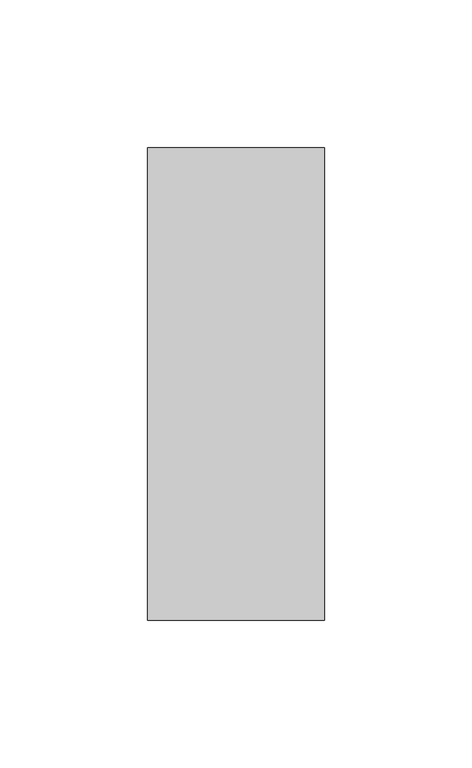
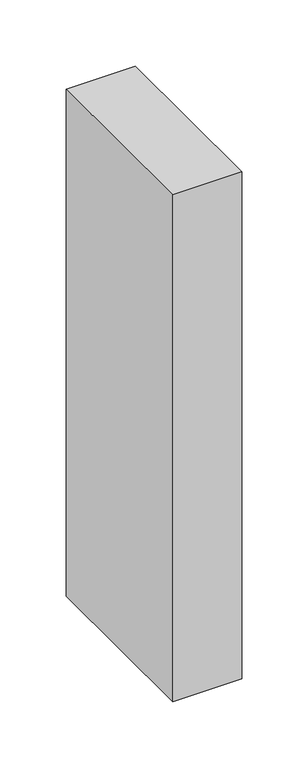
"""IFC4 building model written with IfcOpenShell, lengths in millimetres: column geometry, Madeira de lei-Coluna : Pontalete 6X16cm."""

import ifcopenshell
import ifcopenshell.guid

model = None  # the IFC model being written
_history = None  # IfcOwnerHistory: only IFC2X3 demands one
_inside = {}  # id of a spatial element -> (the spatial element, [elements in it])
_under = {}  # id of a project, library or spatial element -> (it, [spatial elements below it])
_declared = {}  # id of a project -> (the project, [libraries it declares])
_typed = {}  # id of a type object -> (the type object, [elements of that type])
_made_of = {}  # id of a material, layer set ... -> (it, [elements and type objects made of it])


def new_model(schema):
    """Start an empty IFC model of exactly this schema.

    Asked for "IFC4X3", IfcOpenShell would pick the latest addendum, in which some entities
    have other attributes; the version numbers below select the first issue.
    IFC2X3 requires an IfcOwnerHistory on every rooted entity: one is made here for all.
    """
    global model, _history
    if schema == "IFC4X3":
        model = ifcopenshell.file(schema_version=(4, 3, 0, 0))
    else:
        model = ifcopenshell.file(schema=schema)
    _inside.clear()
    _under.clear()
    _declared.clear()
    _typed.clear()
    _made_of.clear()
    _history = None
    if model.schema == "IFC2X3":
        org = make("IfcOrganization", Name="unknown")
        user = make(
            "IfcPersonAndOrganization",
            ThePerson=make("IfcPerson", FamilyName="unknown"),
            TheOrganization=org,
        )
        app = make(
            "IfcApplication",
            ApplicationDeveloper=org,
            Version="unknown",
            ApplicationFullName="unknown",
            ApplicationIdentifier="unknown",
        )
        _history = make(
            "IfcOwnerHistory",
            OwningUser=user,
            OwningApplication=app,
            ChangeAction="ADDED",
            CreationDate=0,
        )
    return model


def make(cls, **values):
    """One entity of the class cls with the attributes given. An attribute that is None is left unset."""
    return model.create_entity(
        cls, **{name: value for name, value in values.items() if value is not None}
    )


def rooted(cls, **values):
    """An entity with a GlobalId (a new one), such as an element, a storey or a relation."""
    return make(cls, GlobalId=ifcopenshell.guid.new(), OwnerHistory=_history, **values)


def si_unit(unit_type, name, prefix=None):
    """IfcSIUnit, for example si_unit("LENGTHUNIT", "METRE", prefix="MILLI")."""
    return make("IfcSIUnit", UnitType=unit_type, Prefix=prefix, Name=name)


def assignment(units):
    """IfcUnitAssignment: the units of a project."""
    return None if units is None else make("IfcUnitAssignment", Units=units)


def point(xyz):
    """IfcCartesianPoint."""
    return None if xyz is None else make("IfcCartesianPoint", Coordinates=xyz)


def direction(xyz):
    """IfcDirection."""
    return None if xyz is None else make("IfcDirection", DirectionRatios=xyz)


def frame(location, z_axis=None, x_axis=None):
    """IfcAxis2Placement3D, a coordinate frame: its origin and axes. An axis left out is left unset."""
    return make(
        "IfcAxis2Placement3D",
        Location=point(location),
        Axis=direction(z_axis),
        RefDirection=direction(x_axis),
    )


def origin():
    """The frame at (0, 0, 0) with its axes left unset."""
    return frame((0.0, 0.0, 0.0))


def place(relative_to, where):
    """IfcLocalPlacement: puts the frame where relative to a parent placement (None: the world)."""
    return make(
        "IfcLocalPlacement", PlacementRelTo=relative_to, RelativePlacement=where
    )


def context(
    kind, dimensions, precision=None, world=None, true_north=None, identifier=None
):
    """IfcGeometricRepresentationContext, for example the 3D "Model" context."""
    return make(
        "IfcGeometricRepresentationContext",
        ContextIdentifier=identifier,
        ContextType=kind,
        CoordinateSpaceDimension=dimensions,
        Precision=precision,
        WorldCoordinateSystem=world,
        TrueNorth=true_north,
    )


def project(units=None, contexts=None):
    """IfcProject with its units and contexts."""
    return rooted(
        "IfcProject",
        Name="project",
        RepresentationContexts=contexts,
        UnitsInContext=assignment(units),
    )


def spatial(cls, under=None, at=None, **own):
    """A site, building, storey or space (cls), placed at a placement, below another one or the project."""
    s = rooted(cls, ObjectPlacement=at, **own)
    if under is not None:
        _under.setdefault(under.id(), (under, []))[1].append(s)
    return s


def polyline(points):
    """IfcPolyline through the points."""
    return make("IfcPolyline", Points=[point(p) for p in points])


def outline(outer, holes=None, kind="AREA"):
    """IfcArbitraryClosedProfileDef: a profile drawn as a closed curve; with holes, ...WithVoids."""
    if holes is None:
        return make("IfcArbitraryClosedProfileDef", ProfileType=kind, OuterCurve=outer)
    return make(
        "IfcArbitraryProfileDefWithVoids",
        ProfileType=kind,
        OuterCurve=outer,
        InnerCurves=holes,
    )


def extrude(swept, where, along, depth):
    """IfcExtrudedAreaSolid: the profile swept, set in the frame where, extruded along a direction by depth."""
    return make(
        "IfcExtrudedAreaSolid",
        SweptArea=swept,
        Position=where,
        ExtrudedDirection=direction(along),
        Depth=depth,
    )


def shape(context_of_items, identifier, shape_type, items):
    """IfcShapeRepresentation: the items that make up one representation, for example the "Body"."""
    return make(
        "IfcShapeRepresentation",
        ContextOfItems=context_of_items,
        RepresentationIdentifier=identifier,
        RepresentationType=shape_type,
        Items=items,
    )


def source(mapping_origin, context_of_items, identifier, shape_type, items):
    """IfcRepresentationMap: a shape defined once, which mapped items show again and again."""
    return make(
        "IfcRepresentationMap",
        MappingOrigin=mapping_origin,
        MappedRepresentation=shape(context_of_items, identifier, shape_type, items),
    )


def transform(
    local_origin,
    x_axis=None,
    y_axis=None,
    z_axis=None,
    scale=None,
    scale2=None,
    scale3=None,
    uniform=True,
):
    """IfcCartesianTransformationOperator3D, or its non-uniform kind. x_axis, y_axis, z_axis: its Axis1, 2, 3."""
    if uniform:
        return make(
            "IfcCartesianTransformationOperator3D",
            Axis1=direction(x_axis),
            Axis2=direction(y_axis),
            LocalOrigin=point(local_origin),
            Scale=scale,
            Axis3=direction(z_axis),
        )
    return make(
        "IfcCartesianTransformationOperator3DnonUniform",
        Axis1=direction(x_axis),
        Axis2=direction(y_axis),
        LocalOrigin=point(local_origin),
        Scale=scale,
        Axis3=direction(z_axis),
        Scale2=scale2,
        Scale3=scale3,
    )


def mapped(mapping_source, mapping_target):
    """IfcMappedItem: shows the shape of a source again, moved by a transform."""
    return make(
        "IfcMappedItem", MappingSource=mapping_source, MappingTarget=mapping_target
    )


def made_of(thing, what):
    """Note that an element or type object is made of a material, layer set ...; save() writes the relation."""
    if what is not None:
        _made_of.setdefault(what.id(), (what, []))[1].append(thing)
    return thing


def element(
    cls,
    number,
    at=None,
    inside=None,
    cuts=None,
    type_object=None,
    material=None,
    context=None,
    identifier="Body",
    shape_type=None,
    held_by="IfcProductDefinitionShape",
    body=None,
    shapes=None,
    **own,
):
    """One element of the class cls, such as IfcWall. Its Tag is "e" and its number.

    at: its placement. inside: the storey or other place that contains it. cuts: it is an
    opening in that element (IfcRelVoidsElement). A single representation is given by context,
    identifier, shape_type and body (its items); several are given by shapes. held_by: the class
    of the entity that holds the representations. save() writes the other relations.
    """
    e = rooted(cls, Tag="e%d" % number, ObjectPlacement=at, **own)
    if body is not None:
        shapes = [shape(context, identifier, shape_type, body)]
    if shapes is not None:
        e.Representation = make(held_by, Representations=shapes)
    if inside is not None:
        _inside.setdefault(inside.id(), (inside, []))[1].append(e)
    if cuts is not None:
        rooted(
            "IfcRelVoidsElement", RelatingBuildingElement=cuts, RelatedOpeningElement=e
        )
    if type_object is not None:
        _typed.setdefault(type_object.id(), (type_object, []))[1].append(e)
    return made_of(e, material)


def aggregate(whole, parts):
    """IfcRelAggregates: a whole, such as a stair, and the parts it consists of."""
    return rooted("IfcRelAggregates", RelatingObject=whole, RelatedObjects=parts)


def save(model, path):
    """Write the relations noted so far, then the file.

    IfcRelAggregates (storeys below a building ...), IfcRelContainedInSpatialStructure (elements
    in a storey), IfcRelDefinesByType, IfcRelAssociatesMaterial and IfcRelDeclares: one each for
    every whole, place, type object, material and project.
    """
    for whole, parts in _under.values():
        aggregate(whole, parts)
    for where, things in _inside.values():
        rooted(
            "IfcRelContainedInSpatialStructure",
            RelatedElements=things,
            RelatingStructure=where,
        )
    for kind, things in _typed.values():
        rooted("IfcRelDefinesByType", RelatedObjects=things, RelatingType=kind)
    for what, things in _made_of.values():
        rooted("IfcRelAssociatesMaterial", RelatedObjects=things, RelatingMaterial=what)
    for by, libraries in _declared.values():
        rooted("IfcRelDeclares", RelatingContext=by, RelatedDefinitions=libraries)
    model.write(path)


def column_7d6827b5(model_context):
    return source(origin(), model_context, "Body", "SweptSolid", [
        extrude(outline(polyline([(30.0, 80.0), (30.0, -80.0), (-30.0, -80.0), (-30.0, 80.0), (30.0, 80.0)])), frame((0.0, 0.0, 4460.0), z_axis=(0.0, 0.0, 1.0), x_axis=(1.0, 0.0, 0.0)), (0.0, 0.0, 1.0), 466.0),
    ])


if __name__ == "__main__":
    model = new_model("IFC4")
    model_context = context("Model", 3, world=origin())
    ifc_project = project(units=[si_unit("LENGTHUNIT", "METRE", prefix="MILLI")], contexts=[model_context])
    site = spatial("IfcSite", under=ifc_project)
    building = spatial("IfcBuilding", under=site)
    placement = place(None, origin())
    column_shape = column_7d6827b5(model_context)
    element("IfcColumn", 1, ObjectType="Madeira de lei-Coluna : Pontalete 6X16cm", at=placement, inside=building, context=model_context, shape_type="MappedRepresentation", body=[
        mapped(column_shape, transform((0.0, 0.0, 0.0), x_axis=(1.0, 0.0, 0.0), y_axis=(0.0, 1.0, 0.0), z_axis=(0.0, 0.0, 1.0))),
    ])
    save(model, "model.ifc")

# Revit data of these elements
# Type "Madeira de lei-Coluna : Pontalete 6X16cm"
#   A = 0.01952 m²
#   b = 0.06 m
#   d = 0.16 m
#   Structural Material [instance default] = none
#   Assembly Code = ""
# Element 1 (IfcColumn, "Madeira de lei-Coluna : Pontalete 6X16cm")
#   Structural Material = .MADEIRAMENTO
#   Materials on its faces: ".MADEIRAMENTO"
# Materials
#   ".MADEIRAMENTO": class ".CC_MADEIRAS", colour RGB 212 179 113, transparency 0, Cost = 0
